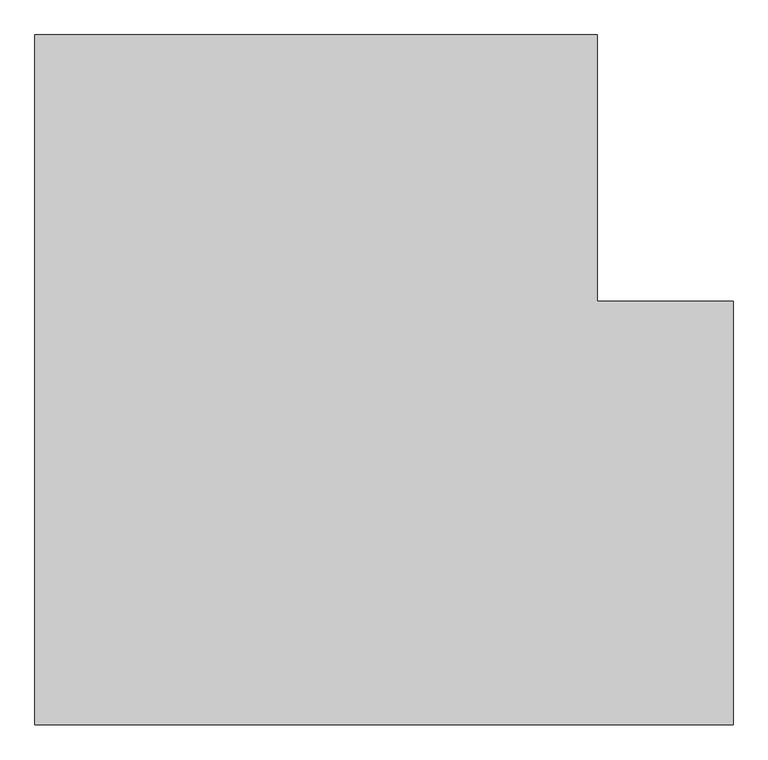
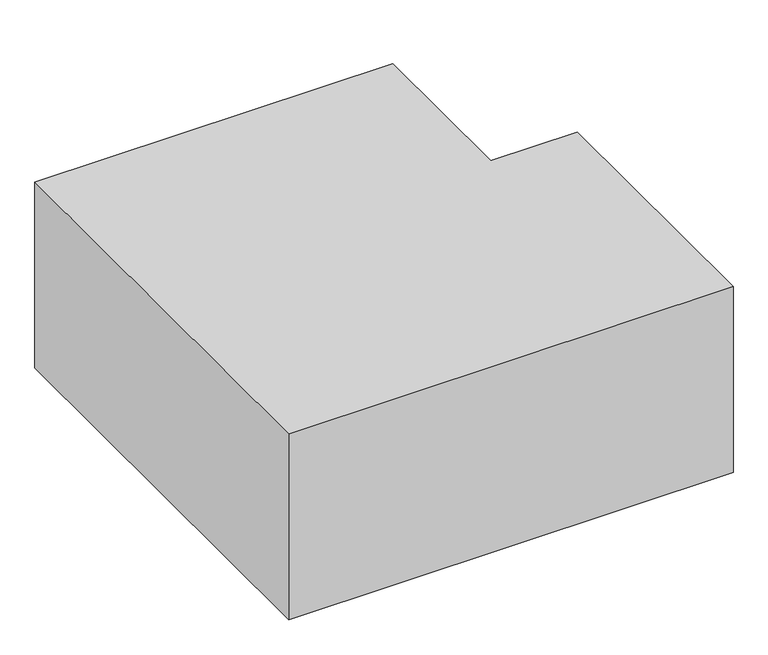
"""IFC4 building model written with IfcOpenShell, lengths in millimetres: proxy geometry, 0_3d_modell."""

import ifcopenshell
import ifcopenshell.guid

model = None  # the IFC model being written
_history = None  # IfcOwnerHistory: only IFC2X3 demands one
_inside = {}  # id of a spatial element -> (the spatial element, [elements in it])
_under = {}  # id of a project, library or spatial element -> (it, [spatial elements below it])
_declared = {}  # id of a project -> (the project, [libraries it declares])
_typed = {}  # id of a type object -> (the type object, [elements of that type])
_made_of = {}  # id of a material, layer set ... -> (it, [elements and type objects made of it])


def new_model(schema):
    """Start an empty IFC model of exactly this schema.

    Asked for "IFC4X3", IfcOpenShell would pick the latest addendum, in which some entities
    have other attributes; the version numbers below select the first issue.
    IFC2X3 requires an IfcOwnerHistory on every rooted entity: one is made here for all.
    """
    global model, _history
    if schema == "IFC4X3":
        model = ifcopenshell.file(schema_version=(4, 3, 0, 0))
    else:
        model = ifcopenshell.file(schema=schema)
    _inside.clear()
    _under.clear()
    _declared.clear()
    _typed.clear()
    _made_of.clear()
    _history = None
    if model.schema == "IFC2X3":
        org = make("IfcOrganization", Name="unknown")
        user = make(
            "IfcPersonAndOrganization",
            ThePerson=make("IfcPerson", FamilyName="unknown"),
            TheOrganization=org,
        )
        app = make(
            "IfcApplication",
            ApplicationDeveloper=org,
            Version="unknown",
            ApplicationFullName="unknown",
            ApplicationIdentifier="unknown",
        )
        _history = make(
            "IfcOwnerHistory",
            OwningUser=user,
            OwningApplication=app,
            ChangeAction="ADDED",
            CreationDate=0,
        )
    return model


def make(cls, **values):
    """One entity of the class cls with the attributes given. An attribute that is None is left unset."""
    return model.create_entity(
        cls, **{name: value for name, value in values.items() if value is not None}
    )


def rooted(cls, **values):
    """An entity with a GlobalId (a new one), such as an element, a storey or a relation."""
    return make(cls, GlobalId=ifcopenshell.guid.new(), OwnerHistory=_history, **values)


def si_unit(unit_type, name, prefix=None):
    """IfcSIUnit, for example si_unit("LENGTHUNIT", "METRE", prefix="MILLI")."""
    return make("IfcSIUnit", UnitType=unit_type, Prefix=prefix, Name=name)


def assignment(units):
    """IfcUnitAssignment: the units of a project."""
    return None if units is None else make("IfcUnitAssignment", Units=units)


def point(xyz):
    """IfcCartesianPoint."""
    return None if xyz is None else make("IfcCartesianPoint", Coordinates=xyz)


def direction(xyz):
    """IfcDirection."""
    return None if xyz is None else make("IfcDirection", DirectionRatios=xyz)


def frame(location, z_axis=None, x_axis=None):
    """IfcAxis2Placement3D, a coordinate frame: its origin and axes. An axis left out is left unset."""
    return make(
        "IfcAxis2Placement3D",
        Location=point(location),
        Axis=direction(z_axis),
        RefDirection=direction(x_axis),
    )


def origin():
    """The frame at (0, 0, 0) with its axes left unset."""
    return frame((0.0, 0.0, 0.0))


def origin_with_axes():
    """The frame at (0, 0, 0) with the z axis (0, 0, 1) and the x axis (1, 0, 0) written out."""
    return frame((0.0, 0.0, 0.0), z_axis=(0.0, 0.0, 1.0), x_axis=(1.0, 0.0, 0.0))


def place(relative_to, where):
    """IfcLocalPlacement: puts the frame where relative to a parent placement (None: the world)."""
    return make(
        "IfcLocalPlacement", PlacementRelTo=relative_to, RelativePlacement=where
    )


def context(
    kind, dimensions, precision=None, world=None, true_north=None, identifier=None
):
    """IfcGeometricRepresentationContext, for example the 3D "Model" context."""
    return make(
        "IfcGeometricRepresentationContext",
        ContextIdentifier=identifier,
        ContextType=kind,
        CoordinateSpaceDimension=dimensions,
        Precision=precision,
        WorldCoordinateSystem=world,
        TrueNorth=true_north,
    )


def project(units=None, contexts=None):
    """IfcProject with its units and contexts."""
    return rooted(
        "IfcProject",
        Name="project",
        RepresentationContexts=contexts,
        UnitsInContext=assignment(units),
    )


def spatial(cls, under=None, at=None, **own):
    """A site, building, storey or space (cls), placed at a placement, below another one or the project."""
    s = rooted(cls, ObjectPlacement=at, **own)
    if under is not None:
        _under.setdefault(under.id(), (under, []))[1].append(s)
    return s


def polyline(points):
    """IfcPolyline through the points."""
    return make("IfcPolyline", Points=[point(p) for p in points])


def outline(outer, holes=None, kind="AREA"):
    """IfcArbitraryClosedProfileDef: a profile drawn as a closed curve; with holes, ...WithVoids."""
    if holes is None:
        return make("IfcArbitraryClosedProfileDef", ProfileType=kind, OuterCurve=outer)
    return make(
        "IfcArbitraryProfileDefWithVoids",
        ProfileType=kind,
        OuterCurve=outer,
        InnerCurves=holes,
    )


def extrude(swept, where, along, depth):
    """IfcExtrudedAreaSolid: the profile swept, set in the frame where, extruded along a direction by depth."""
    return make(
        "IfcExtrudedAreaSolid",
        SweptArea=swept,
        Position=where,
        ExtrudedDirection=direction(along),
        Depth=depth,
    )


def shape(context_of_items, identifier, shape_type, items):
    """IfcShapeRepresentation: the items that make up one representation, for example the "Body"."""
    return make(
        "IfcShapeRepresentation",
        ContextOfItems=context_of_items,
        RepresentationIdentifier=identifier,
        RepresentationType=shape_type,
        Items=items,
    )


def source(mapping_origin, context_of_items, identifier, shape_type, items):
    """IfcRepresentationMap: a shape defined once, which mapped items show again and again."""
    return make(
        "IfcRepresentationMap",
        MappingOrigin=mapping_origin,
        MappedRepresentation=shape(context_of_items, identifier, shape_type, items),
    )


def transform(
    local_origin,
    x_axis=None,
    y_axis=None,
    z_axis=None,
    scale=None,
    scale2=None,
    scale3=None,
    uniform=True,
):
    """IfcCartesianTransformationOperator3D, or its non-uniform kind. x_axis, y_axis, z_axis: its Axis1, 2, 3."""
    if uniform:
        return make(
            "IfcCartesianTransformationOperator3D",
            Axis1=direction(x_axis),
            Axis2=direction(y_axis),
            LocalOrigin=point(local_origin),
            Scale=scale,
            Axis3=direction(z_axis),
        )
    return make(
        "IfcCartesianTransformationOperator3DnonUniform",
        Axis1=direction(x_axis),
        Axis2=direction(y_axis),
        LocalOrigin=point(local_origin),
        Scale=scale,
        Axis3=direction(z_axis),
        Scale2=scale2,
        Scale3=scale3,
    )


def mapped(mapping_source, mapping_target):
    """IfcMappedItem: shows the shape of a source again, moved by a transform."""
    return make(
        "IfcMappedItem", MappingSource=mapping_source, MappingTarget=mapping_target
    )


def made_of(thing, what):
    """Note that an element or type object is made of a material, layer set ...; save() writes the relation."""
    if what is not None:
        _made_of.setdefault(what.id(), (what, []))[1].append(thing)
    return thing


def element(
    cls,
    number,
    at=None,
    inside=None,
    cuts=None,
    type_object=None,
    material=None,
    context=None,
    identifier="Body",
    shape_type=None,
    held_by="IfcProductDefinitionShape",
    body=None,
    shapes=None,
    **own,
):
    """One element of the class cls, such as IfcWall. Its Tag is "e" and its number.

    at: its placement. inside: the storey or other place that contains it. cuts: it is an
    opening in that element (IfcRelVoidsElement). A single representation is given by context,
    identifier, shape_type and body (its items); several are given by shapes. held_by: the class
    of the entity that holds the representations. save() writes the other relations.
    """
    e = rooted(cls, Tag="e%d" % number, ObjectPlacement=at, **own)
    if body is not None:
        shapes = [shape(context, identifier, shape_type, body)]
    if shapes is not None:
        e.Representation = make(held_by, Representations=shapes)
    if inside is not None:
        _inside.setdefault(inside.id(), (inside, []))[1].append(e)
    if cuts is not None:
        rooted(
            "IfcRelVoidsElement", RelatingBuildingElement=cuts, RelatedOpeningElement=e
        )
    if type_object is not None:
        _typed.setdefault(type_object.id(), (type_object, []))[1].append(e)
    return made_of(e, material)


def aggregate(whole, parts):
    """IfcRelAggregates: a whole, such as a stair, and the parts it consists of."""
    return rooted("IfcRelAggregates", RelatingObject=whole, RelatedObjects=parts)


def save(model, path):
    """Write the relations noted so far, then the file.

    IfcRelAggregates (storeys below a building ...), IfcRelContainedInSpatialStructure (elements
    in a storey), IfcRelDefinesByType, IfcRelAssociatesMaterial and IfcRelDeclares: one each for
    every whole, place, type object, material and project.
    """
    for whole, parts in _under.values():
        aggregate(whole, parts)
    for where, things in _inside.values():
        rooted(
            "IfcRelContainedInSpatialStructure",
            RelatedElements=things,
            RelatingStructure=where,
        )
    for kind, things in _typed.values():
        rooted("IfcRelDefinesByType", RelatedObjects=things, RelatingType=kind)
    for what, things in _made_of.values():
        rooted("IfcRelAssociatesMaterial", RelatedObjects=things, RelatingMaterial=what)
    for by, libraries in _declared.values():
        rooted("IfcRelDeclares", RelatingContext=by, RelatedDefinitions=libraries)
    model.write(path)


def generic_models_805eeb56(model_context):
    return source(origin(), model_context, "Body", "SweptSolid", [
        extrude(outline(polyline([(5650.0, 3427.8619019), (5649.840708, 0.0), (0.0, 0.0), (0.0, 5582.8619019), (4550.0, 5582.8619019), (4550.0, 3427.8619019), (5650.0, 3427.8619019)])), origin_with_axes(), (0.0, 0.0, 1.0), 2500.0),
    ])


if __name__ == "__main__":
    model = new_model("IFC4")
    model_context = context("Model", 3, world=origin())
    ifc_project = project(units=[si_unit("LENGTHUNIT", "METRE", prefix="MILLI")], contexts=[model_context])
    site = spatial("IfcSite", under=ifc_project)
    building = spatial("IfcBuilding", under=site)
    placement = place(None, origin())
    generic_models_shape = generic_models_805eeb56(model_context)
    element("IfcBuildingElementProxy", 1, Name="0_3d_modell", ObjectType="0_3d_modell", at=placement, inside=building, context=model_context, shape_type="MappedRepresentation", body=[
        mapped(generic_models_shape, transform((0.0, 0.0, 0.0), x_axis=(1.0, 0.0, 0.0), y_axis=(0.0, 1.0, 0.0), z_axis=(0.0, 0.0, 1.0))),
    ])
    save(model, "model.ifc")

# Revit data of these elements
# Element 1 (IfcBuildingElementProxy, "0_3d_modell")
#   Materials on its faces: "*1"
# Materials
#   "*1": class "Unassigned", colour RGB 175 175 175, transparency 0
